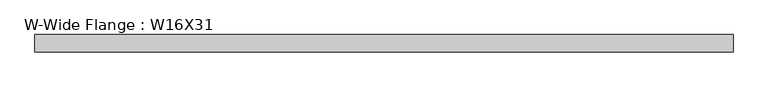
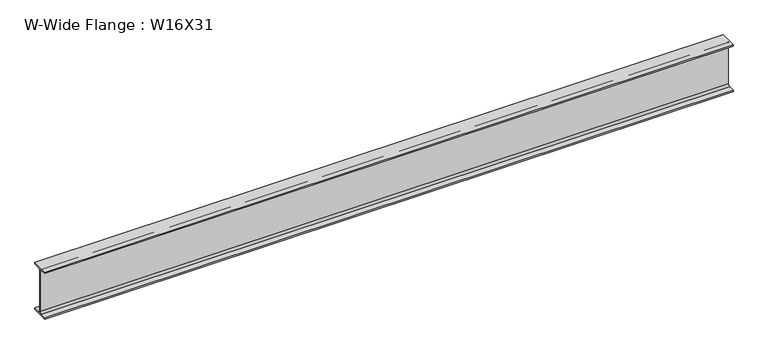
"""IFC4 building model written with IfcOpenShell, lengths in millimetres: beam geometry, W-Wide Flange : W16X31."""

from ifc_helpers import new_model, si_unit, point, frame, frame_2d, origin, place, context, project, spatial, polyline, circle_curve, trimmed, segment, composite_curve, outline, extrude, source, transform, mapped, element, save


def w_wide_flange_w16x31_9ce748ab(model_context):
    return source(origin(), model_context, "Body", "SweptSolid", [
        extrude(outline(composite_curve([segment(polyline([(70.231, -190.754), (70.231, -201.93), (-70.231, -201.93), (-70.231, -190.754), (-20.8915, -190.754)]), True, "CONTINUOUS"), segment(trimmed(circle_curve(frame_2d((-20.8915, -173.355)), 17.399), [point((-20.8915, -190.754))], [point((-3.4925, -173.355))], True, "CARTESIAN"), True, "CONTINUOUS"), segment(polyline([(-3.4925, -173.355), (-3.4925, 173.355)]), True, "CONTINUOUS"), segment(trimmed(circle_curve(frame_2d((-20.8915, 173.355)), 17.399), [point((-3.4925, 173.355))], [point((-20.8915, 190.754))], True, "CARTESIAN"), True, "CONTINUOUS"), segment(polyline([(-20.8915, 190.754), (-70.231, 190.754), (-70.231, 201.93), (70.231, 201.93), (70.231, 190.754), (20.8915, 190.754)]), True, "CONTINUOUS"), segment(trimmed(circle_curve(frame_2d((20.8915, 173.355)), 17.399), [point((20.8915, 190.754))], [point((3.4925, 173.355))], True, "CARTESIAN"), True, "CONTINUOUS"), segment(polyline([(3.4925, 173.355), (3.4925, -173.355)]), True, "CONTINUOUS"), segment(trimmed(circle_curve(frame_2d((20.8915, -173.355)), 17.399), [point((3.4925, -173.355))], [point((20.8915, -190.754))], True, "CARTESIAN"), True, "CONTINUOUS"), segment(polyline([(20.8915, -190.754), (70.231, -190.754)]), True, "CONTINUOUS")], self_intersect=False)), frame((-2806.7, 0.0, 0.0), z_axis=(1.0, 0.0, 0.0), x_axis=(0.0, 1.0, 0.0)), (0.0, 0.0, 1.0), 5613.4),
    ])


if __name__ == "__main__":
    model = new_model("IFC4")
    model_context = context("Model", 3, world=origin())
    ifc_project = project(units=[si_unit("LENGTHUNIT", "METRE", prefix="MILLI")], contexts=[model_context])
    site = spatial("IfcSite", under=ifc_project)
    building = spatial("IfcBuilding", under=site)
    placement = place(None, origin())
    w_wide_flange_w16x31_shape = w_wide_flange_w16x31_9ce748ab(model_context)
    element("IfcBeam", 1, ObjectType="W-Wide Flange : W16X31", at=placement, inside=building, context=model_context, shape_type="MappedRepresentation", body=[
        mapped(w_wide_flange_w16x31_shape, transform((0.0, 0.0, 0.0), x_axis=(1.0, 0.0, 0.0), y_axis=(0.0, 1.0, 0.0), z_axis=(0.0, 0.0, 1.0))),
    ])
    save(model, "model.ifc")

# Revit data of these elements
# Type "W-Wide Flange : W16X31"
#   Assembly Code = "B10"
#   W = 31
#   Length [instance default] = 5' - 0"
#   bf = 0' - 5.53"
#   d = 1' - 3.9"
#   k = 0' - 1 1/8"
#   k2 = 0' - 0.685"
#   tf = 0' - 0.44"
#   tw = 0' - 0.275"
#   A = 0.0634028 SF
#   Structural Material [instance default] = Steel ASTM A992
# Element 1 (IfcBeam, "W-Wide Flange : W16X31")
#   Materials on its faces: "Steel ASTM A992"
# Materials
#   "Steel ASTM A992": class "Metal", colour RGB 199 199 199, transparency 0, Description = "Structural steel 50ksi", Cost = 0
